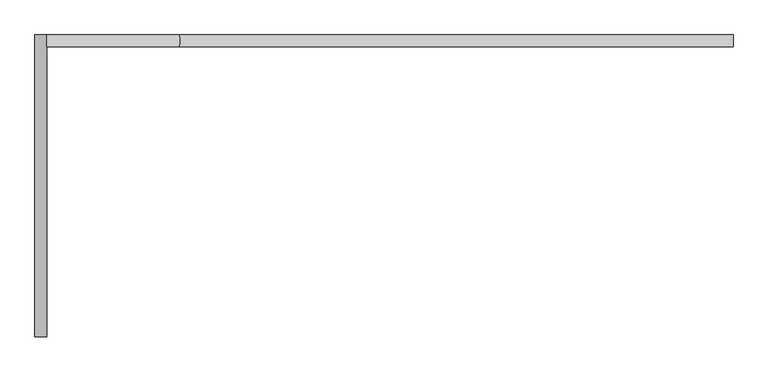
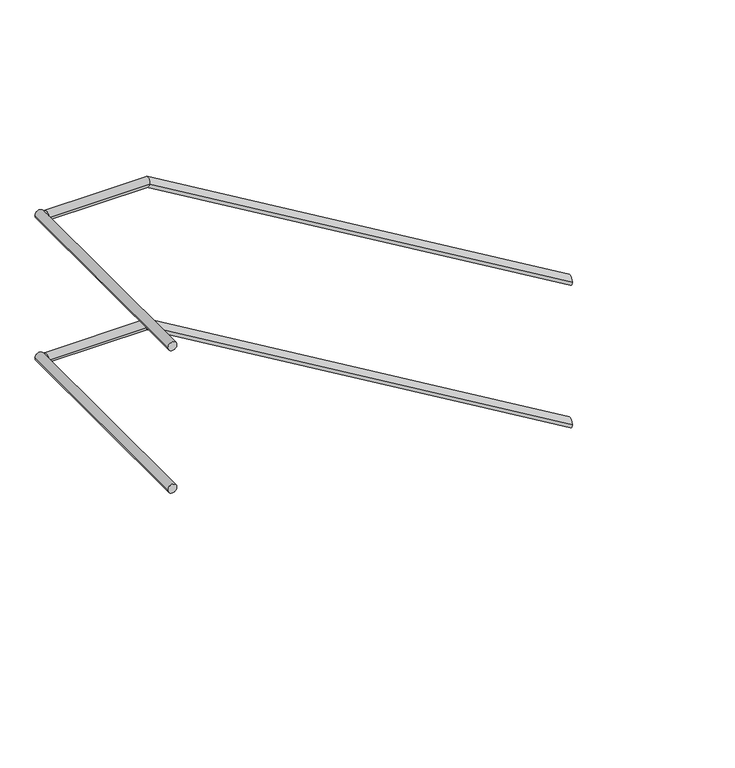
"""IFC4 building model written with IfcOpenShell, lengths in millimetres: railing geometry."""

import ifcopenshell
import ifcopenshell.guid

model = None  # the IFC model being written
_history = None  # IfcOwnerHistory: only IFC2X3 demands one
_inside = {}  # id of a spatial element -> (the spatial element, [elements in it])
_under = {}  # id of a project, library or spatial element -> (it, [spatial elements below it])
_declared = {}  # id of a project -> (the project, [libraries it declares])
_typed = {}  # id of a type object -> (the type object, [elements of that type])
_made_of = {}  # id of a material, layer set ... -> (it, [elements and type objects made of it])


def new_model(schema):
    """Start an empty IFC model of exactly this schema.

    Asked for "IFC4X3", IfcOpenShell would pick the latest addendum, in which some entities
    have other attributes; the version numbers below select the first issue.
    IFC2X3 requires an IfcOwnerHistory on every rooted entity: one is made here for all.
    """
    global model, _history
    if schema == "IFC4X3":
        model = ifcopenshell.file(schema_version=(4, 3, 0, 0))
    else:
        model = ifcopenshell.file(schema=schema)
    _inside.clear()
    _under.clear()
    _declared.clear()
    _typed.clear()
    _made_of.clear()
    _history = None
    if model.schema == "IFC2X3":
        org = make("IfcOrganization", Name="unknown")
        user = make(
            "IfcPersonAndOrganization",
            ThePerson=make("IfcPerson", FamilyName="unknown"),
            TheOrganization=org,
        )
        app = make(
            "IfcApplication",
            ApplicationDeveloper=org,
            Version="unknown",
            ApplicationFullName="unknown",
            ApplicationIdentifier="unknown",
        )
        _history = make(
            "IfcOwnerHistory",
            OwningUser=user,
            OwningApplication=app,
            ChangeAction="ADDED",
            CreationDate=0,
        )
    return model


def make(cls, **values):
    """One entity of the class cls with the attributes given. An attribute that is None is left unset."""
    return model.create_entity(
        cls, **{name: value for name, value in values.items() if value is not None}
    )


def rooted(cls, **values):
    """An entity with a GlobalId (a new one), such as an element, a storey or a relation."""
    return make(cls, GlobalId=ifcopenshell.guid.new(), OwnerHistory=_history, **values)


def si_unit(unit_type, name, prefix=None):
    """IfcSIUnit, for example si_unit("LENGTHUNIT", "METRE", prefix="MILLI")."""
    return make("IfcSIUnit", UnitType=unit_type, Prefix=prefix, Name=name)


def assignment(units):
    """IfcUnitAssignment: the units of a project."""
    return None if units is None else make("IfcUnitAssignment", Units=units)


def point(xyz):
    """IfcCartesianPoint."""
    return None if xyz is None else make("IfcCartesianPoint", Coordinates=xyz)


def direction(xyz):
    """IfcDirection."""
    return None if xyz is None else make("IfcDirection", DirectionRatios=xyz)


def frame(location, z_axis=None, x_axis=None):
    """IfcAxis2Placement3D, a coordinate frame: its origin and axes. An axis left out is left unset."""
    return make(
        "IfcAxis2Placement3D",
        Location=point(location),
        Axis=direction(z_axis),
        RefDirection=direction(x_axis),
    )


def origin():
    """The frame at (0, 0, 0) with its axes left unset."""
    return frame((0.0, 0.0, 0.0))


def place(relative_to, where):
    """IfcLocalPlacement: puts the frame where relative to a parent placement (None: the world)."""
    return make(
        "IfcLocalPlacement", PlacementRelTo=relative_to, RelativePlacement=where
    )


def context(
    kind, dimensions, precision=None, world=None, true_north=None, identifier=None
):
    """IfcGeometricRepresentationContext, for example the 3D "Model" context."""
    return make(
        "IfcGeometricRepresentationContext",
        ContextIdentifier=identifier,
        ContextType=kind,
        CoordinateSpaceDimension=dimensions,
        Precision=precision,
        WorldCoordinateSystem=world,
        TrueNorth=true_north,
    )


def project(units=None, contexts=None):
    """IfcProject with its units and contexts."""
    return rooted(
        "IfcProject",
        Name="project",
        RepresentationContexts=contexts,
        UnitsInContext=assignment(units),
    )


def spatial(cls, under=None, at=None, **own):
    """A site, building, storey or space (cls), placed at a placement, below another one or the project."""
    s = rooted(cls, ObjectPlacement=at, **own)
    if under is not None:
        _under.setdefault(under.id(), (under, []))[1].append(s)
    return s


def circle_curve(where, radius):
    """IfcCircle in the frame where."""
    return make("IfcCircle", Position=where, Radius=radius)


def ellipse_curve(where, semi_axis1, semi_axis2):
    """IfcEllipse in the frame where."""
    return make(
        "IfcEllipse", Position=where, SemiAxis1=semi_axis1, SemiAxis2=semi_axis2
    )


def shape(context_of_items, identifier, shape_type, items):
    """IfcShapeRepresentation: the items that make up one representation, for example the "Body"."""
    return make(
        "IfcShapeRepresentation",
        ContextOfItems=context_of_items,
        RepresentationIdentifier=identifier,
        RepresentationType=shape_type,
        Items=items,
    )


def source(mapping_origin, context_of_items, identifier, shape_type, items):
    """IfcRepresentationMap: a shape defined once, which mapped items show again and again."""
    return make(
        "IfcRepresentationMap",
        MappingOrigin=mapping_origin,
        MappedRepresentation=shape(context_of_items, identifier, shape_type, items),
    )


def transform(
    local_origin,
    x_axis=None,
    y_axis=None,
    z_axis=None,
    scale=None,
    scale2=None,
    scale3=None,
    uniform=True,
):
    """IfcCartesianTransformationOperator3D, or its non-uniform kind. x_axis, y_axis, z_axis: its Axis1, 2, 3."""
    if uniform:
        return make(
            "IfcCartesianTransformationOperator3D",
            Axis1=direction(x_axis),
            Axis2=direction(y_axis),
            LocalOrigin=point(local_origin),
            Scale=scale,
            Axis3=direction(z_axis),
        )
    return make(
        "IfcCartesianTransformationOperator3DnonUniform",
        Axis1=direction(x_axis),
        Axis2=direction(y_axis),
        LocalOrigin=point(local_origin),
        Scale=scale,
        Axis3=direction(z_axis),
        Scale2=scale2,
        Scale3=scale3,
    )


def mapped(mapping_source, mapping_target):
    """IfcMappedItem: shows the shape of a source again, moved by a transform."""
    return make(
        "IfcMappedItem", MappingSource=mapping_source, MappingTarget=mapping_target
    )


def made_of(thing, what):
    """Note that an element or type object is made of a material, layer set ...; save() writes the relation."""
    if what is not None:
        _made_of.setdefault(what.id(), (what, []))[1].append(thing)
    return thing


def element(
    cls,
    number,
    at=None,
    inside=None,
    cuts=None,
    type_object=None,
    material=None,
    context=None,
    identifier="Body",
    shape_type=None,
    held_by="IfcProductDefinitionShape",
    body=None,
    shapes=None,
    **own,
):
    """One element of the class cls, such as IfcWall. Its Tag is "e" and its number.

    at: its placement. inside: the storey or other place that contains it. cuts: it is an
    opening in that element (IfcRelVoidsElement). A single representation is given by context,
    identifier, shape_type and body (its items); several are given by shapes. held_by: the class
    of the entity that holds the representations. save() writes the other relations.
    """
    e = rooted(cls, Tag="e%d" % number, ObjectPlacement=at, **own)
    if body is not None:
        shapes = [shape(context, identifier, shape_type, body)]
    if shapes is not None:
        e.Representation = make(held_by, Representations=shapes)
    if inside is not None:
        _inside.setdefault(inside.id(), (inside, []))[1].append(e)
    if cuts is not None:
        rooted(
            "IfcRelVoidsElement", RelatingBuildingElement=cuts, RelatedOpeningElement=e
        )
    if type_object is not None:
        _typed.setdefault(type_object.id(), (type_object, []))[1].append(e)
    return made_of(e, material)


def aggregate(whole, parts):
    """IfcRelAggregates: a whole, such as a stair, and the parts it consists of."""
    return rooted("IfcRelAggregates", RelatingObject=whole, RelatedObjects=parts)


def save(model, path):
    """Write the relations noted so far, then the file.

    IfcRelAggregates (storeys below a building ...), IfcRelContainedInSpatialStructure (elements
    in a storey), IfcRelDefinesByType, IfcRelAssociatesMaterial and IfcRelDeclares: one each for
    every whole, place, type object, material and project.
    """
    for whole, parts in _under.values():
        aggregate(whole, parts)
    for where, things in _inside.values():
        rooted(
            "IfcRelContainedInSpatialStructure",
            RelatedElements=things,
            RelatingStructure=where,
        )
    for kind, things in _typed.values():
        rooted("IfcRelDefinesByType", RelatedObjects=things, RelatingType=kind)
    for what, things in _made_of.values():
        rooted("IfcRelAssociatesMaterial", RelatedObjects=things, RelatingMaterial=what)
    for by, libraries in _declared.values():
        rooted("IfcRelDeclares", RelatingContext=by, RelatedDefinitions=libraries)
    model.write(path)


def plane_surface(at):
    """IfcPlane: the flat surface through the origin of the frame at, square to its z axis."""
    return make("IfcPlane", Position=at)


def cylinder_surface(at, radius):
    """IfcCylindricalSurface: all points at the distance radius from the z axis of the frame at."""
    return make("IfcCylindricalSurface", Position=at, Radius=radius)


def advanced_brep(points, edges, surfaces, faces):
    """IfcAdvancedBrep: a solid bounded by faces that lie on surfaces and meet in shared edges.

    An edge is (start, end): straight between two places in points (the first is 0);
    or (start, end, curve); or (start, end, curve, False) where it runs against its curve.
    A face is (place in surfaces, loops), or (place, loops, False) where it looks against
    its surface's normal. A loop lists edges by number (the first is 1), with a minus sign
    where the edge is run from its end to its start. The first loop is the outer one.
    """
    corners = [point(p) for p in points]
    vertices = [make("IfcVertexPoint", VertexGeometry=c) for c in corners]
    made = []
    for start, end, *more in edges:
        made.append(
            make(
                "IfcEdgeCurve",
                EdgeStart=vertices[start],
                EdgeEnd=vertices[end],
                EdgeGeometry=more[0] if more else make("IfcPolyline", Points=[corners[start], corners[end]]),
                SameSense=more[1] if len(more) > 1 else True,
            )
        )
    hull = []
    for where, loops, *sense in faces:
        bounds = []
        for j, loop in enumerate(loops):
            ring = [make("IfcOrientedEdge", EdgeElement=made[abs(k) - 1], Orientation=k > 0) for k in loop]
            bounds.append(
                make(
                    "IfcFaceOuterBound" if j == 0 else "IfcFaceBound",
                    Bound=make("IfcEdgeLoop", EdgeList=ring),
                    Orientation=True,
                )
            )
        hull.append(make("IfcAdvancedFace", Bounds=bounds, FaceSurface=surfaces[where], SameSense=sense[0] if sense else True))
    return make("IfcAdvancedBrep", Outer=make("IfcClosedShell", CfsFaces=hull))


def railing_0945bab5(model_context):
    return source(origin(), model_context, "Body", "AdvancedBrep", [
        advanced_brep(
        [(33043.8956602, 24484.5208589, 899.1723166), (33043.8956602, 24514.5208589, 899.1723166), (31639.7692216, 24484.5208589, 1734.9618634), (31639.7692216, 24514.5208589, 1734.9618634), (31305.4, 24484.5208589, 1734.9618634), (31305.4, 24514.5208589, 1734.9618634)],
        [
            (0, 1, ellipse_curve(frame((33043.8956602, 24499.5208589, 899.1723166), z_axis=(1.0, 0.0, 0.0), x_axis=(0.0, 0.0, -1.0)), 17.4562134, 15.0)),
            (1, 0, ellipse_curve(frame((33043.8956602, 24499.5208589, 899.1723166), z_axis=(1.0, 0.0, 0.0), x_axis=(0.0, 0.0, -1.0)), 17.4562134, 15.0)),
            (0, 2),
            (2, 3, ellipse_curve(frame((31639.7692216, 24499.5208589, 1734.9618634), z_axis=(0.9641817474962141, 0.0, -0.2652424509673118), x_axis=(-0.26524245096731197, 0.0, -0.9641817474962142)), 15.5572329, 15.0)),
            (3, 1),
            (3, 2, ellipse_curve(frame((31639.7692216, 24499.5208589, 1734.9618634), z_axis=(0.9641817474962141, 0.0, -0.2652424509673118), x_axis=(-0.26524245096731197, 0.0, -0.9641817474962142)), 15.5572329, 15.0)),
            (4, 5, circle_curve(frame((31305.4, 24499.5208589, 1734.9618634), z_axis=(-1.0, 0.0, 0.0), x_axis=(0.0, 1.0, 0.0)), 15.0)),
            (5, 4, circle_curve(frame((31305.4, 24499.5208589, 1734.9618634), z_axis=(-1.0, 0.0, 0.0), x_axis=(0.0, 1.0, 0.0)), 15.0)),
            (2, 4),
            (5, 3),
        ],
        [
            plane_surface(frame((33043.8956602, 24499.5208589, 916.62853), z_axis=(1.0, 0.0, 0.0), x_axis=(0.0, -1.0, 0.0))),
            cylinder_surface(frame((33036.2234023, 24499.5208589, 903.7391368), z_axis=(0.8592928844097064, 0.0, -0.5114838597676832), x_axis=(0.0, 1.0, 0.0)), 15.0),
            plane_surface(frame((31305.4, 24499.5208589, 1749.9618634), z_axis=(-1.0, 0.0, 0.0), x_axis=(0.0, -1.0, 0.0))),
            cylinder_surface(frame((31643.8956602, 24499.5208589, 1734.9618634), z_axis=(1.0, 0.0, 0.0), x_axis=(0.0, 1.0, 0.0)), 15.0),
        ],
        [
            (0, [[1, 2]]),
            (1, [[-1, 3, 4, 5]]),
            (1, [[-2, -5, 6, -3]]),
            (2, [[7, 8]]),
            (3, [[-4, 9, -8, 10]]),
            (3, [[-6, -10, -7, -9]]),
        ],
    ),
        advanced_brep(
        [(33043.8956602, 24484.5208589, 1399.1723166), (33043.8956602, 24514.5208589, 1399.1723166), (31639.7692216, 24484.5208589, 2234.9618634), (31639.7692216, 24514.5208589, 2234.9618634), (31305.4, 24484.5208589, 2234.9618634), (31305.4, 24514.5208589, 2234.9618634)],
        [
            (0, 1, ellipse_curve(frame((33043.8956602, 24499.5208589, 1399.1723166), z_axis=(1.0, 0.0, 0.0), x_axis=(0.0, 0.0, -1.0)), 17.4562134, 15.0)),
            (1, 0, ellipse_curve(frame((33043.8956602, 24499.5208589, 1399.1723166), z_axis=(1.0, 0.0, 0.0), x_axis=(0.0, 0.0, -1.0)), 17.4562134, 15.0)),
            (0, 2),
            (2, 3, ellipse_curve(frame((31639.7692216, 24499.5208589, 2234.9618634), z_axis=(0.9641817474962141, 0.0, -0.2652424509673118), x_axis=(-0.26524245096731197, 0.0, -0.9641817474962142)), 15.5572329, 15.0)),
            (3, 1),
            (3, 2, ellipse_curve(frame((31639.7692216, 24499.5208589, 2234.9618634), z_axis=(0.9641817474962141, 0.0, -0.2652424509673118), x_axis=(-0.26524245096731197, 0.0, -0.9641817474962142)), 15.5572329, 15.0)),
            (4, 5, circle_curve(frame((31305.4, 24499.5208589, 2234.9618634), z_axis=(-1.0, 0.0, 0.0), x_axis=(0.0, 1.0, 0.0)), 15.0)),
            (5, 4, circle_curve(frame((31305.4, 24499.5208589, 2234.9618634), z_axis=(-1.0, 0.0, 0.0), x_axis=(0.0, 1.0, 0.0)), 15.0)),
            (2, 4),
            (5, 3),
        ],
        [
            plane_surface(frame((33043.8956602, 24499.5208589, 1416.62853), z_axis=(1.0, 0.0, 0.0), x_axis=(0.0, -1.0, 0.0))),
            cylinder_surface(frame((33036.2234023, 24499.5208589, 1403.7391368), z_axis=(0.8592928844097064, 0.0, -0.5114838597676832), x_axis=(0.0, 1.0, 0.0)), 15.0),
            plane_surface(frame((31305.4, 24499.5208589, 2249.9618634), z_axis=(-1.0, 0.0, 0.0), x_axis=(0.0, -1.0, 0.0))),
            cylinder_surface(frame((31643.8956602, 24499.5208589, 2234.9618634), z_axis=(1.0, 0.0, 0.0), x_axis=(0.0, 1.0, 0.0)), 15.0),
        ],
        [
            (0, [[1, 2]]),
            (1, [[-1, 3, 4, 5]]),
            (1, [[-2, -5, 6, -3]]),
            (2, [[7, 8]]),
            (3, [[-4, 9, -8, 10]]),
            (3, [[-6, -10, -7, -9]]),
        ],
    ),
        advanced_brep(
        [(31305.4, 24514.5208589, 1734.9618634), (31275.4, 24514.5208589, 1734.9618634), (31305.4, 23749.5208589, 1734.9618634), (31275.4, 23749.5208589, 1734.9618634)],
        [
            (0, 1, circle_curve(frame((31290.4, 24514.5208589, 1734.9618634), z_axis=(0.0, 1.0, 0.0), x_axis=(-1.0, 0.0, 0.0)), 15.0)),
            (1, 0, circle_curve(frame((31290.4, 24514.5208589, 1734.9618634), z_axis=(0.0, 1.0, 0.0), x_axis=(-1.0, 0.0, 0.0)), 15.0)),
            (2, 3, circle_curve(frame((31290.4, 23749.5208589, 1734.9618634), z_axis=(0.0, -1.0, 0.0), x_axis=(-1.0, 0.0, 0.0)), 15.0)),
            (3, 2, circle_curve(frame((31290.4, 23749.5208589, 1734.9618634), z_axis=(0.0, -1.0, 0.0), x_axis=(-1.0, 0.0, 0.0)), 15.0)),
            (0, 2),
            (3, 1),
        ],
        [
            plane_surface(frame((31290.4, 24514.5208589, 1749.9618634), z_axis=(0.0, 1.0, 0.0), x_axis=(0.0, 0.0, -1.0))),
            plane_surface(frame((31290.4, 23749.5208589, 1749.9618634), z_axis=(0.0, -1.0, 0.0), x_axis=(0.0, 0.0, -1.0))),
            cylinder_surface(frame((31290.4, 24514.5208589, 1734.9618634), z_axis=(0.0, 1.0, 0.0), x_axis=(-1.0, 0.0, 0.0)), 15.0),
        ],
        [
            (0, [[1, 2]]),
            (1, [[3, 4]]),
            (2, [[-1, 5, -4, 6]]),
            (2, [[-2, -6, -3, -5]]),
        ],
    ),
        advanced_brep(
        [(31305.4, 24514.5208589, 2234.9618634), (31275.4, 24514.5208589, 2234.9618634), (31305.4, 23749.5208589, 2234.9618634), (31275.4, 23749.5208589, 2234.9618634)],
        [
            (0, 1, circle_curve(frame((31290.4, 24514.5208589, 2234.9618634), z_axis=(0.0, 1.0, 0.0), x_axis=(-1.0, 0.0, 0.0)), 15.0)),
            (1, 0, circle_curve(frame((31290.4, 24514.5208589, 2234.9618634), z_axis=(0.0, 1.0, 0.0), x_axis=(-1.0, 0.0, 0.0)), 15.0)),
            (2, 3, circle_curve(frame((31290.4, 23749.5208589, 2234.9618634), z_axis=(0.0, -1.0, 0.0), x_axis=(-1.0, 0.0, 0.0)), 15.0)),
            (3, 2, circle_curve(frame((31290.4, 23749.5208589, 2234.9618634), z_axis=(0.0, -1.0, 0.0), x_axis=(-1.0, 0.0, 0.0)), 15.0)),
            (0, 2),
            (3, 1),
        ],
        [
            plane_surface(frame((31290.4, 24514.5208589, 2249.9618634), z_axis=(0.0, 1.0, 0.0), x_axis=(0.0, 0.0, -1.0))),
            plane_surface(frame((31290.4, 23749.5208589, 2249.9618634), z_axis=(0.0, -1.0, 0.0), x_axis=(0.0, 0.0, -1.0))),
            cylinder_surface(frame((31290.4, 24514.5208589, 2234.9618634), z_axis=(0.0, 1.0, 0.0), x_axis=(-1.0, 0.0, 0.0)), 15.0),
        ],
        [
            (0, [[1, 2]]),
            (1, [[3, 4]]),
            (2, [[-1, 5, -4, 6]]),
            (2, [[-2, -6, -3, -5]]),
        ],
    ),
    ])


if __name__ == "__main__":
    model = new_model("IFC4")
    model_context = context("Model", 3, world=origin())
    ifc_project = project(units=[si_unit("LENGTHUNIT", "METRE", prefix="MILLI")], contexts=[model_context])
    site = spatial("IfcSite", under=ifc_project)
    building = spatial("IfcBuilding", under=site)
    placement = place(None, origin())
    railing_shape = railing_0945bab5(model_context)
    element("IfcRailing", 1, at=placement, inside=building, context=model_context, shape_type="MappedRepresentation", body=[
        mapped(railing_shape, transform((0.0, 0.0, 0.0), x_axis=(1.0, 0.0, 0.0), y_axis=(0.0, 1.0, 0.0), z_axis=(0.0, 0.0, 1.0))),
    ])
    save(model, "model.ifc")
